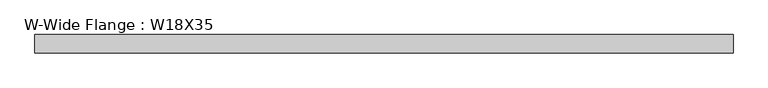
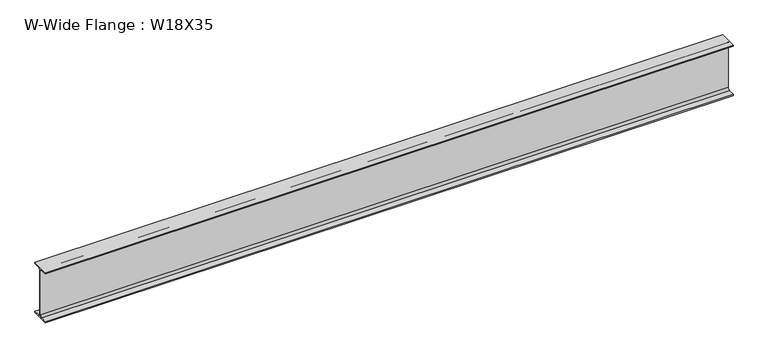
"""IFC4 building model written with IfcOpenShell, lengths in millimetres: beam geometry, W-Wide Flange : W18X35."""

from ifc_helpers import new_model, si_unit, point, frame, frame_2d, origin, place, context, project, spatial, polyline, circle_curve, trimmed, segment, composite_curve, outline, extrude, source, transform, mapped, element, save


def w_wide_flange_w18x35_f828bc5f(model_context):
    return source(origin(), model_context, "Body", "SweptSolid", [
        extrude(outline(composite_curve([segment(polyline([(76.2, -213.995), (76.2, -224.79), (-76.2, -224.79), (-76.2, -213.995), (-21.59, -213.995)]), True, "CONTINUOUS"), segment(trimmed(circle_curve(frame_2d((-21.59, -196.215)), 17.78), [point((-21.59, -213.995))], [point((-3.81, -196.215))], True, "CARTESIAN"), True, "CONTINUOUS"), segment(polyline([(-3.81, -196.215), (-3.81, 196.215)]), True, "CONTINUOUS"), segment(trimmed(circle_curve(frame_2d((-21.59, 196.215)), 17.78), [point((-3.81, 196.215))], [point((-21.59, 213.995))], True, "CARTESIAN"), True, "CONTINUOUS"), segment(polyline([(-21.59, 213.995), (-76.2, 213.995), (-76.2, 224.79), (76.2, 224.79), (76.2, 213.995), (21.59, 213.995)]), True, "CONTINUOUS"), segment(trimmed(circle_curve(frame_2d((21.59, 196.215)), 17.78), [point((21.59, 213.995))], [point((3.81, 196.215))], True, "CARTESIAN"), True, "CONTINUOUS"), segment(polyline([(3.81, 196.215), (3.81, -196.215)]), True, "CONTINUOUS"), segment(trimmed(circle_curve(frame_2d((21.59, -196.215)), 17.78), [point((3.81, -196.215))], [point((21.59, -213.995))], True, "CARTESIAN"), True, "CONTINUOUS"), segment(polyline([(21.59, -213.995), (76.2, -213.995)]), True, "CONTINUOUS")], self_intersect=False)), frame((-2908.3, 0.0, 0.0), z_axis=(1.0, 0.0, 0.0), x_axis=(0.0, 1.0, 0.0)), (0.0, 0.0, 1.0), 5816.6),
    ])


if __name__ == "__main__":
    model = new_model("IFC4")
    model_context = context("Model", 3, world=origin())
    ifc_project = project(units=[si_unit("LENGTHUNIT", "METRE", prefix="MILLI")], contexts=[model_context])
    site = spatial("IfcSite", under=ifc_project)
    building = spatial("IfcBuilding", under=site)
    placement = place(None, origin())
    w_wide_flange_w18x35_shape = w_wide_flange_w18x35_f828bc5f(model_context)
    element("IfcBeam", 1, ObjectType="W-Wide Flange : W18X35", at=placement, inside=building, context=model_context, shape_type="MappedRepresentation", body=[
        mapped(w_wide_flange_w18x35_shape, transform((0.0, 0.0, 0.0), x_axis=(1.0, 0.0, 0.0), y_axis=(0.0, 1.0, 0.0), z_axis=(0.0, 0.0, 1.0))),
    ])
    save(model, "model.ifc")

# Revit data of these elements
# Type "W-Wide Flange : W18X35"
#   Assembly Code = "B10"
#   W = 35
#   Length [instance default] = 5' - 0"
#   bf = 0' - 6"
#   d = 1' - 5.7"
#   k = 0' - 1 1/8"
#   k2 = 0' - 0.7"
#   tf = 0' - 0.425"
#   tw = 0' - 0.3"
#   A = 0.0715278 SF
#   Structural Material [instance default] = Steel ASTM A992
# Element 1 (IfcBeam, "W-Wide Flange : W18X35")
#   Materials on its faces: "Steel ASTM A992"
# Materials
#   "Steel ASTM A992": class "Metal", colour RGB 199 199 199, transparency 0, Description = "Structural steel 50ksi", Cost = 0
